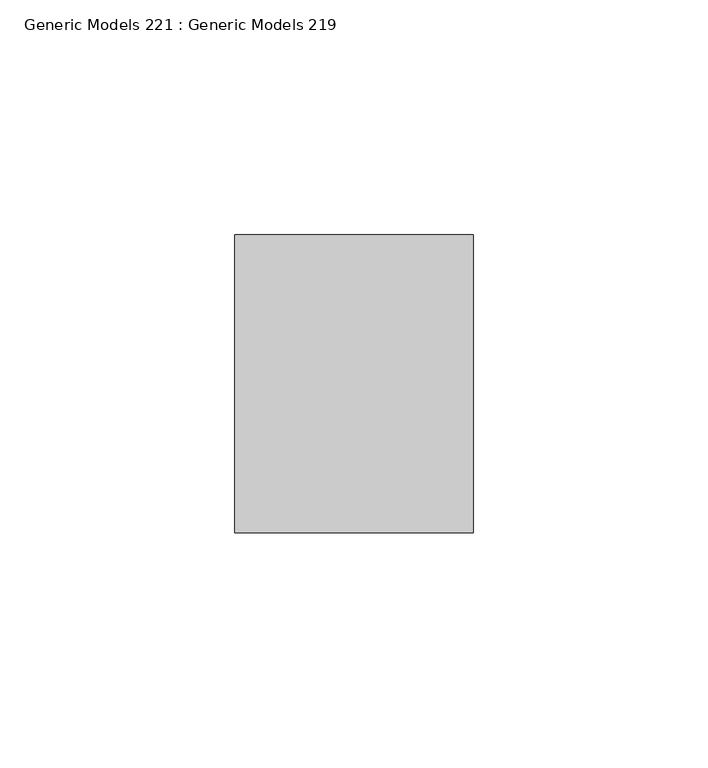
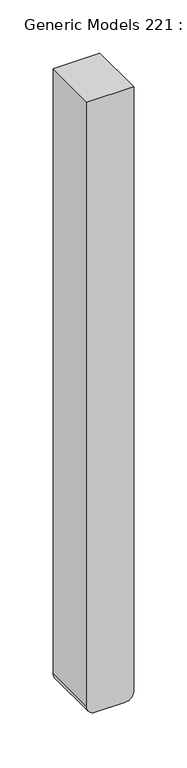
"""IFC4 building model written with IfcOpenShell, lengths in millimetres: proxy geometry, Generic Models 221 : Generic Models 219."""

from ifc_helpers import new_model, si_unit, point, frame, frame_2d, origin, place, context, project, spatial, polyline, circle_curve, trimmed, segment, composite_curve, outline, extrude, source, transform, mapped, element, save


def generic_models_221_generic_models_219_cf3d814a(model_context):
    return source(origin(), model_context, "Body", "SweptSolid", [
        extrude(outline(composite_curve([segment(trimmed(circle_curve(frame_2d((123712.9352, 7838.2155704)), 8.8392), [point((123712.9352, 7829.3763704))], [point((123704.096, 7838.2155704))], False, "CARTESIAN"), True, "CONTINUOUS"), segment(polyline([(123704.096, 7838.2155704), (123704.096, 7871.3371704)]), True, "CONTINUOUS"), segment(trimmed(circle_curve(frame_2d((123712.9352, 7871.3371704)), 8.8392), [point((123704.096, 7871.3371704))], [point((123712.9352, 7880.1763704))], False, "CARTESIAN"), True, "CONTINUOUS"), segment(polyline([(123712.9352, 7880.1763704), (124408.5606599, 7880.1763704), (124408.5606599, 7829.3763704), (123712.9352, 7829.3763704)]), True, "CONTINUOUS")], self_intersect=False)), frame((0.0, 4501.3863946, 0.0), z_axis=(0.0, 1.0, 0.0), x_axis=(0.0, 0.0, 1.0)), (0.0, 0.0, 1.0), 63.500874),
    ])


if __name__ == "__main__":
    model = new_model("IFC4")
    model_context = context("Model", 3, world=origin())
    ifc_project = project(units=[si_unit("LENGTHUNIT", "METRE", prefix="MILLI")], contexts=[model_context])
    site = spatial("IfcSite", under=ifc_project)
    building = spatial("IfcBuilding", under=site)
    placement = place(None, origin())
    generic_models_221_generic_models_219_shape = generic_models_221_generic_models_219_cf3d814a(model_context)
    element("IfcBuildingElementProxy", 1, Name="Generic Models 221 : Generic Models 219", ObjectType="Generic Models 221 : Generic Models 219", at=placement, inside=building, context=model_context, shape_type="MappedRepresentation", body=[
        mapped(generic_models_221_generic_models_219_shape, transform((0.0, 0.0, 0.0), x_axis=(1.0, 0.0, 0.0), y_axis=(0.0, 1.0, 0.0), z_axis=(0.0, 0.0, 1.0))),
    ])
    save(model, "model.ifc")

# Revit data of these elements
# Element 1 (IfcBuildingElementProxy, "Generic Models 221 : Generic Models 219")
#   Materials on its faces: "_2x3 STEEL PROFILE - METALIZED, PRIMED & PAINTED (COLOR PER ARCHITECT)"
# Materials
#   "_2x3 STEEL PROFILE - METALIZED, PRIMED & PAINTED (COLOR PER ARCHITECT)": class "Metal", colour RGB 199 199 199, transparency 0, Description = "Structural steel 50ksi", Cost = 0
